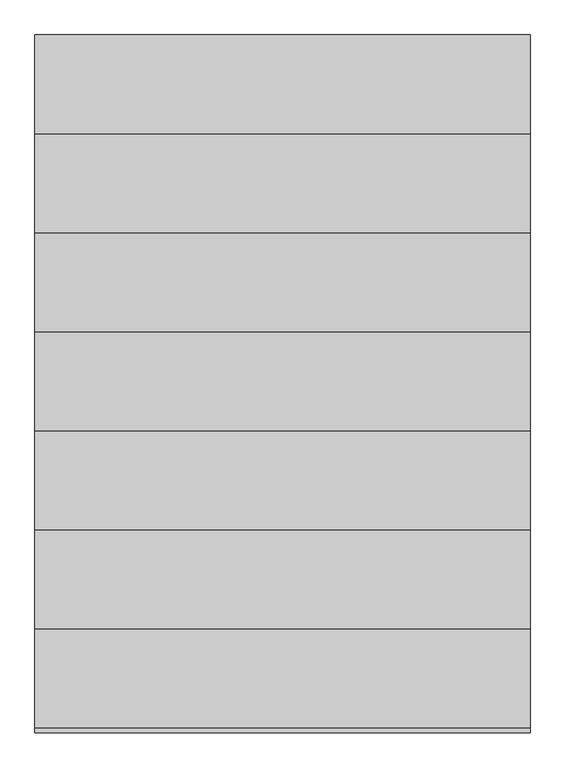
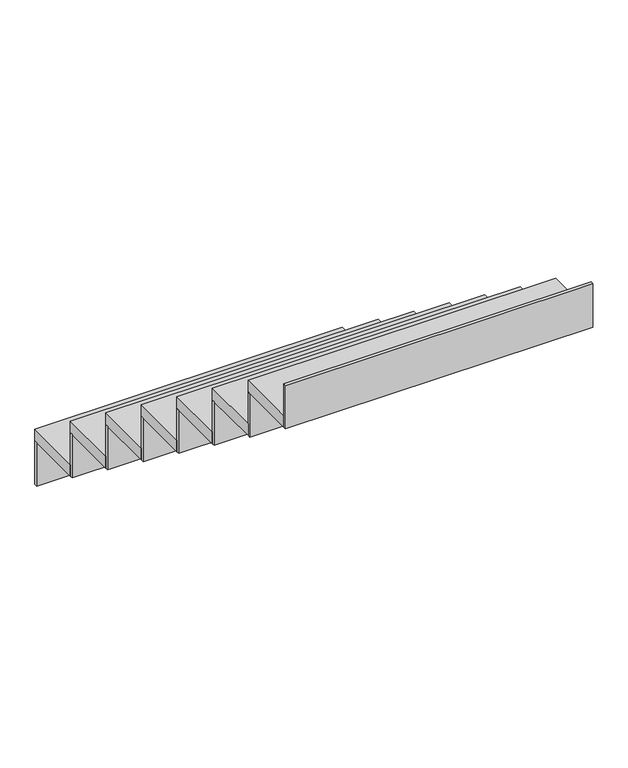
"""IFC4 building model written with IfcOpenShell, lengths in millimetres: stair flight geometry."""

from ifc_helpers import new_model, si_unit, frame, origin, place, context, project, spatial, polyline, outline, extrude, source, transform, mapped, element, save


def stair_flight_2d2a652e(model_context):
    return source(origin(), model_context, "Body", "SweptSolid", [
        extrude(outline(polyline([(-11830.6631644, -9565.1519052), (-11830.6631644, -9552.6519052), (-10580.6631644, -9552.6519052), (-10580.6631644, -9565.1519052), (-11830.6631644, -9565.1519052)])), frame((0.0, 0.0, 1443.3333333), z_axis=(0.0, 0.0, 1.0), x_axis=(1.0, 0.0, 0.0)), (0.0, 0.0, 1.0), 186.6666667),
        extrude(outline(polyline([(-10580.6631644, -9802.6519052), (-11830.6631644, -9802.6519052), (-11830.6631644, -9552.6519052), (-10580.6631644, -9552.6519052), (-10580.6631644, -9802.6519052)])), frame((0.0, 0.0, 1630.0), z_axis=(0.0, 0.0, 1.0), x_axis=(1.0, 0.0, 0.0)), (0.0, 0.0, 1.0), 50.0),
        extrude(outline(polyline([(-11830.6631644, -9815.1519052), (-11830.6631644, -9802.6519052), (-10580.6631644, -9802.6519052), (-10580.6631644, -9815.1519052), (-11830.6631644, -9815.1519052)])), frame((0.0, 0.0, 1630.0), z_axis=(0.0, 0.0, 1.0), x_axis=(1.0, 0.0, 0.0)), (0.0, 0.0, 1.0), 186.6666667),
        extrude(outline(polyline([(-10580.6631644, -10052.6519052), (-11830.6631644, -10052.6519052), (-11830.6631644, -9802.6519052), (-10580.6631644, -9802.6519052), (-10580.6631644, -10052.6519052)])), frame((0.0, 0.0, 1816.6666667), z_axis=(0.0, 0.0, 1.0), x_axis=(1.0, 0.0, 0.0)), (0.0, 0.0, 1.0), 50.0),
        extrude(outline(polyline([(-11830.6631644, -10065.1519052), (-11830.6631644, -10052.6519052), (-10580.6631644, -10052.6519052), (-10580.6631644, -10065.1519052), (-11830.6631644, -10065.1519052)])), frame((0.0, 0.0, 1816.6666667), z_axis=(0.0, 0.0, 1.0), x_axis=(1.0, 0.0, 0.0)), (0.0, 0.0, 1.0), 186.6666667),
        extrude(outline(polyline([(-10580.6631644, -10302.6519052), (-11830.6631644, -10302.6519052), (-11830.6631644, -10052.6519052), (-10580.6631644, -10052.6519052), (-10580.6631644, -10302.6519052)])), frame((0.0, 0.0, 2003.3333333), z_axis=(0.0, 0.0, 1.0), x_axis=(1.0, 0.0, 0.0)), (0.0, 0.0, 1.0), 50.0),
        extrude(outline(polyline([(-11830.6631644, -10315.1519052), (-11830.6631644, -10302.6519052), (-10580.6631644, -10302.6519052), (-10580.6631644, -10315.1519052), (-11830.6631644, -10315.1519052)])), frame((0.0, 0.0, 2003.3333333), z_axis=(0.0, 0.0, 1.0), x_axis=(1.0, 0.0, 0.0)), (0.0, 0.0, 1.0), 186.6666667),
        extrude(outline(polyline([(-10580.6631644, -10552.6519052), (-11830.6631644, -10552.6519052), (-11830.6631644, -10302.6519052), (-10580.6631644, -10302.6519052), (-10580.6631644, -10552.6519052)])), frame((0.0, 0.0, 2190.0), z_axis=(0.0, 0.0, 1.0), x_axis=(1.0, 0.0, 0.0)), (0.0, 0.0, 1.0), 50.0),
        extrude(outline(polyline([(-11830.6631644, -10565.1519052), (-11830.6631644, -10552.6519052), (-10580.6631644, -10552.6519052), (-10580.6631644, -10565.1519052), (-11830.6631644, -10565.1519052)])), frame((0.0, 0.0, 2190.0), z_axis=(0.0, 0.0, 1.0), x_axis=(1.0, 0.0, 0.0)), (0.0, 0.0, 1.0), 186.6666667),
        extrude(outline(polyline([(-10580.6631644, -10802.6519052), (-11830.6631644, -10802.6519052), (-11830.6631644, -10552.6519052), (-10580.6631644, -10552.6519052), (-10580.6631644, -10802.6519052)])), frame((0.0, 0.0, 2376.6666667), z_axis=(0.0, 0.0, 1.0), x_axis=(1.0, 0.0, 0.0)), (0.0, 0.0, 1.0), 50.0),
        extrude(outline(polyline([(-11830.6631644, -10815.1519052), (-11830.6631644, -10802.6519052), (-10580.6631644, -10802.6519052), (-10580.6631644, -10815.1519052), (-11830.6631644, -10815.1519052)])), frame((0.0, 0.0, 2376.6666667), z_axis=(0.0, 0.0, 1.0), x_axis=(1.0, 0.0, 0.0)), (0.0, 0.0, 1.0), 186.6666667),
        extrude(outline(polyline([(-10580.6631644, -11052.6519052), (-11830.6631644, -11052.6519052), (-11830.6631644, -10802.6519052), (-10580.6631644, -10802.6519052), (-10580.6631644, -11052.6519052)])), frame((0.0, 0.0, 2563.3333333), z_axis=(0.0, 0.0, 1.0), x_axis=(1.0, 0.0, 0.0)), (0.0, 0.0, 1.0), 50.0),
        extrude(outline(polyline([(-11830.6631644, -11065.1519052), (-11830.6631644, -11052.6519052), (-10580.6631644, -11052.6519052), (-10580.6631644, -11065.1519052), (-11830.6631644, -11065.1519052)])), frame((0.0, 0.0, 2563.3333333), z_axis=(0.0, 0.0, 1.0), x_axis=(1.0, 0.0, 0.0)), (0.0, 0.0, 1.0), 186.6666667),
        extrude(outline(polyline([(-11830.6631644, -11315.1519052), (-11830.6631644, -11302.6519052), (-10580.6631644, -11302.6519052), (-10580.6631644, -11315.1519052), (-11830.6631644, -11315.1519052)])), frame((0.0, 0.0, 2750.0), z_axis=(0.0, 0.0, 1.0), x_axis=(1.0, 0.0, 0.0)), (0.0, 0.0, 1.0), 186.6666667),
        extrude(outline(polyline([(-10580.6631644, -11302.6519052), (-11830.6631644, -11302.6519052), (-11830.6631644, -11052.6519052), (-10580.6631644, -11052.6519052), (-10580.6631644, -11302.6519052)])), frame((0.0, 0.0, 2750.0), z_axis=(0.0, 0.0, 1.0), x_axis=(1.0, 0.0, 0.0)), (0.0, 0.0, 1.0), 50.0),
    ])


if __name__ == "__main__":
    model = new_model("IFC4")
    model_context = context("Model", 3, world=origin())
    ifc_project = project(units=[si_unit("LENGTHUNIT", "METRE", prefix="MILLI")], contexts=[model_context])
    site = spatial("IfcSite", under=ifc_project)
    building = spatial("IfcBuilding", under=site)
    placement = place(None, origin())
    stair_flight_shape = stair_flight_2d2a652e(model_context)
    element("IfcStairFlight", 1, at=placement, inside=building, context=model_context, shape_type="MappedRepresentation", body=[
        mapped(stair_flight_shape, transform((0.0, 0.0, 0.0), x_axis=(1.0, 0.0, 0.0), y_axis=(0.0, 1.0, 0.0), z_axis=(0.0, 0.0, 1.0))),
    ])
    save(model, "model.ifc")
